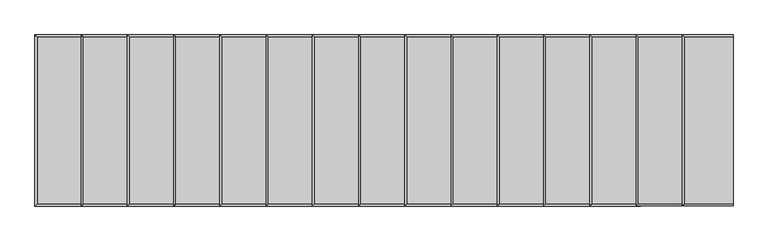
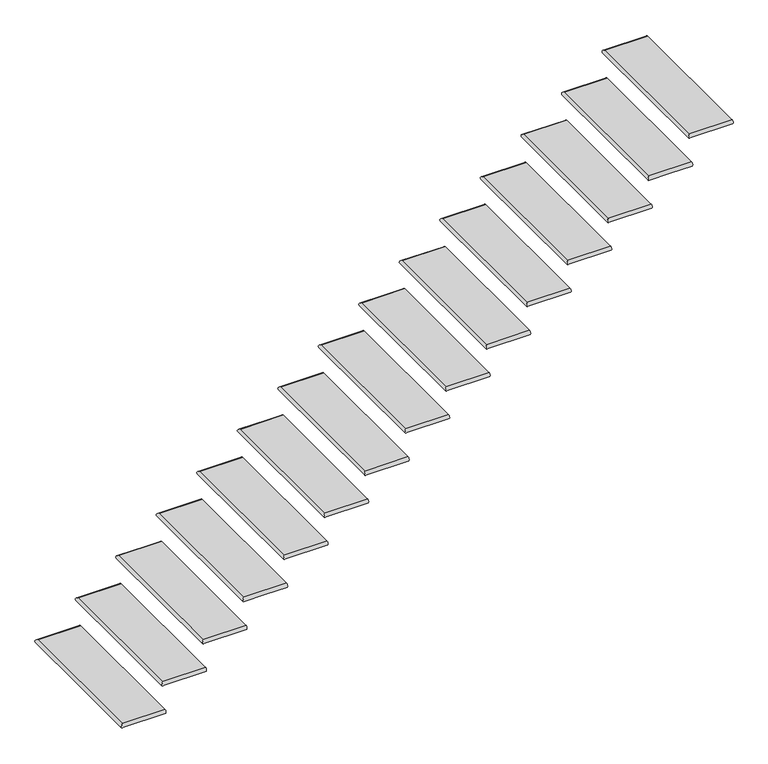
"""IFC4 building model written with IfcOpenShell, lengths in millimetres: stair flight geometry."""

from ifc_helpers import new_model, si_unit, frame, origin, place, context, project, spatial, circle_curve, ellipse_curve, source, transform, mapped, element, save
from ifc_brep_helpers import plane_surface, cylinder_surface, advanced_brep


def stair_flight_3500c2e6(model_context):
    return source(origin(), model_context, "Body", "AdvancedBrep", [
        advanced_brep(
        [(-27218.1481446, -8236.0871906, 165.1), (-27218.1481446, -8236.0871906, 190.5), (-27218.1481446, -7321.6871906, 190.5), (-27218.1481446, -7321.6871906, 165.1), (-26951.4481446, -8236.0871906, 190.5), (-26951.4481446, -7321.6871906, 190.5), (-26951.4481446, -7321.6871906, 165.1), (-26951.4481446, -8236.0871906, 165.1)],
        [
            (0, 1, ellipse_curve(frame((-27218.1481446, -8236.0871906, 177.8), z_axis=(-0.7071067811865464, 0.7071067811865488, 0.0), x_axis=(-0.7071067811865489, -0.707106781186546, 0.0)), 17.9605122, 12.7)),
            (1, 2),
            (2, 3, ellipse_curve(frame((-27218.1481446, -7321.6871906, 177.8), z_axis=(-0.7071067811865487, -0.7071067811865462, 0.0), x_axis=(0.7071067811865462, -0.707106781186549, 0.0)), 17.9605122, 12.7)),
            (3, 0),
            (4, 5),
            (5, 2),
            (1, 4),
            (6, 7),
            (7, 0),
            (3, 6),
            (4, 7, circle_curve(frame((-26951.4481446, -8236.0871906, 177.8), z_axis=(1.0, 0.0, 0.0), x_axis=(0.0, 1.0, 0.0)), 12.7)),
            (6, 5, circle_curve(frame((-26951.4481446, -7321.6871906, 177.8), z_axis=(1.0, 0.0, 0.0), x_axis=(0.0, -1.0, 0.0)), 12.7)),
        ],
        [
            cylinder_surface(frame((-27218.1481446, -8236.0871906, 177.8), z_axis=(0.0, -1.0, 0.0), x_axis=(1.0, 0.0, 0.0)), 12.7),
            plane_surface(frame((-27230.8481446, -7321.6871906, 190.5), z_axis=(0.0, 0.0, 1.0), x_axis=(-1.0, 0.0, 0.0))),
            plane_surface(frame((-27230.8481446, -7321.6871906, 165.1), z_axis=(0.0, 0.0, -1.0), x_axis=(1.0, 0.0, 0.0))),
            plane_surface(frame((-26951.4481446, -8236.0871906, 190.5), z_axis=(1.0, 0.0, 0.0), x_axis=(0.0, 0.0, -1.0))),
            cylinder_surface(frame((-26951.4481446, -8236.0871906, 177.8), z_axis=(1.0, 0.0, 0.0), x_axis=(0.0, 1.0, 0.0)), 12.7),
            cylinder_surface(frame((-27218.1481446, -7321.6871906, 177.8), z_axis=(-1.0, 0.0, 0.0), x_axis=(0.0, -1.0, 0.0)), 12.7),
        ],
        [
            (0, [[1, 2, 3, 4]]),
            (1, [[5, 6, -2, 7]]),
            (2, [[8, 9, -4, 10]]),
            (3, [[-5, 11, -8, 12]]),
            (4, [[-11, -7, -1, -9]]),
            (5, [[-3, -6, -12, -10]]),
        ],
    ),
        advanced_brep(
        [(-26697.4481446, -8236.0871906, 381.0), (-26697.4481446, -7321.6871906, 381.0), (-26964.1481446, -7321.6871906, 381.0), (-26964.1481446, -8236.0871906, 381.0), (-26697.4481446, -7321.6871906, 355.6), (-26697.4481446, -8236.0871906, 355.6), (-26964.1481446, -8236.0871906, 355.6), (-26964.1481446, -7321.6871906, 355.6)],
        [
            (0, 1),
            (1, 2),
            (2, 3),
            (3, 0),
            (4, 5),
            (5, 6),
            (6, 7),
            (7, 4),
            (0, 5, circle_curve(frame((-26697.4481446, -8236.0871906, 368.3), z_axis=(1.0, 0.0, 0.0), x_axis=(0.0, 1.0, 0.0)), 12.7)),
            (4, 1, circle_curve(frame((-26697.4481446, -7321.6871906, 368.3), z_axis=(1.0, 0.0, 0.0), x_axis=(0.0, -1.0, 0.0)), 12.7)),
            (3, 6, ellipse_curve(frame((-26964.1481446, -8236.0871906, 368.3), z_axis=(0.7071067811865464, -0.7071067811865488, 0.0), x_axis=(0.7071067811865487, 0.7071067811865464, 0.0)), 17.9605122, 12.7)),
            (2, 7, ellipse_curve(frame((-26964.1481446, -7321.6871906, 368.3), z_axis=(-0.7071067811865487, -0.7071067811865462, 0.0), x_axis=(0.7071067811865462, -0.707106781186549, 0.0)), 17.9605122, 12.7)),
        ],
        [
            plane_surface(frame((-26976.8481446, -7321.6871906, 381.0), z_axis=(0.0, 0.0, 1.0), x_axis=(-1.0, 0.0, 0.0))),
            plane_surface(frame((-26976.8481446, -7321.6871906, 355.6), z_axis=(0.0, 0.0, -1.0), x_axis=(1.0, 0.0, 0.0))),
            plane_surface(frame((-26697.4481446, -8236.0871906, 381.0), z_axis=(1.0, 0.0, 0.0), x_axis=(0.0, 0.0, -1.0))),
            cylinder_surface(frame((-26697.4481446, -8236.0871906, 368.3), z_axis=(1.0, 0.0, 0.0), x_axis=(0.0, 1.0, 0.0)), 12.7),
            cylinder_surface(frame((-26964.1481446, -8236.0871906, 368.3), z_axis=(0.0, -1.0, 0.0), x_axis=(1.0, 0.0, 0.0)), 12.7),
            cylinder_surface(frame((-26964.1481446, -7321.6871906, 368.3), z_axis=(-1.0, 0.0, 0.0), x_axis=(0.0, -1.0, 0.0)), 12.7),
        ],
        [
            (0, [[1, 2, 3, 4]]),
            (1, [[5, 6, 7, 8]]),
            (2, [[-1, 9, -5, 10]]),
            (3, [[-9, -4, 11, -6]]),
            (4, [[-11, -3, 12, -7]]),
            (5, [[-12, -2, -10, -8]]),
        ],
    ),
        advanced_brep(
        [(-26443.4481446, -8236.0871906, 571.5), (-26443.4481446, -7321.6871906, 571.5), (-26710.1481446, -7321.6871906, 571.5), (-26710.1481446, -8236.0871906, 571.5), (-26443.4481446, -7321.6871906, 546.1), (-26443.4481446, -8236.0871906, 546.1), (-26710.1481446, -8236.0871906, 546.1), (-26710.1481446, -7321.6871906, 546.1)],
        [
            (0, 1),
            (1, 2),
            (2, 3),
            (3, 0),
            (4, 5),
            (5, 6),
            (6, 7),
            (7, 4),
            (0, 5, circle_curve(frame((-26443.4481446, -8236.0871906, 558.8), z_axis=(1.0, 0.0, 0.0), x_axis=(0.0, 1.0, 0.0)), 12.7)),
            (4, 1, circle_curve(frame((-26443.4481446, -7321.6871906, 558.8), z_axis=(1.0, 0.0, 0.0), x_axis=(0.0, -1.0, 0.0)), 12.7)),
            (3, 6, ellipse_curve(frame((-26710.1481446, -8236.0871906, 558.8), z_axis=(0.7071067811865464, -0.7071067811865488, 0.0), x_axis=(0.7071067811865487, 0.7071067811865464, 0.0)), 17.9605122, 12.7)),
            (2, 7, ellipse_curve(frame((-26710.1481446, -7321.6871906, 558.8), z_axis=(-0.7071067811865487, -0.7071067811865462, 0.0), x_axis=(0.7071067811865462, -0.707106781186549, 0.0)), 17.9605122, 12.7)),
        ],
        [
            plane_surface(frame((-26722.8481446, -7321.6871906, 571.5), z_axis=(0.0, 0.0, 1.0), x_axis=(-1.0, 0.0, 0.0))),
            plane_surface(frame((-26722.8481446, -7321.6871906, 546.1), z_axis=(0.0, 0.0, -1.0), x_axis=(1.0, 0.0, 0.0))),
            plane_surface(frame((-26443.4481446, -8236.0871906, 571.5), z_axis=(1.0, 0.0, 0.0), x_axis=(0.0, 0.0, -1.0))),
            cylinder_surface(frame((-26443.4481446, -8236.0871906, 558.8), z_axis=(1.0, 0.0, 0.0), x_axis=(0.0, 1.0, 0.0)), 12.7),
            cylinder_surface(frame((-26710.1481446, -8236.0871906, 558.8), z_axis=(0.0, -1.0, 0.0), x_axis=(1.0, 0.0, 0.0)), 12.7),
            cylinder_surface(frame((-26710.1481446, -7321.6871906, 558.8), z_axis=(-1.0, 0.0, 0.0), x_axis=(0.0, -1.0, 0.0)), 12.7),
        ],
        [
            (0, [[1, 2, 3, 4]]),
            (1, [[5, 6, 7, 8]]),
            (2, [[-1, 9, -5, 10]]),
            (3, [[-9, -4, 11, -6]]),
            (4, [[-11, -3, 12, -7]]),
            (5, [[-12, -2, -10, -8]]),
        ],
    ),
        advanced_brep(
        [(-26189.4481446, -8236.0871906, 762.0), (-26189.4481446, -7321.6871906, 762.0), (-26456.1481446, -7321.6871906, 762.0), (-26456.1481446, -8236.0871906, 762.0), (-26189.4481446, -7321.6871906, 736.6), (-26189.4481446, -8236.0871906, 736.6), (-26456.1481446, -8236.0871906, 736.6), (-26456.1481446, -7321.6871906, 736.6)],
        [
            (0, 1),
            (1, 2),
            (2, 3),
            (3, 0),
            (4, 5),
            (5, 6),
            (6, 7),
            (7, 4),
            (0, 5, circle_curve(frame((-26189.4481446, -8236.0871906, 749.3), z_axis=(1.0, 0.0, 0.0), x_axis=(0.0, 1.0, 0.0)), 12.7)),
            (4, 1, circle_curve(frame((-26189.4481446, -7321.6871906, 749.3), z_axis=(1.0, 0.0, 0.0), x_axis=(0.0, -1.0, 0.0)), 12.7)),
            (3, 6, ellipse_curve(frame((-26456.1481446, -8236.0871906, 749.3), z_axis=(0.7071067811865464, -0.7071067811865488, 0.0), x_axis=(0.7071067811865487, 0.7071067811865464, 0.0)), 17.9605122, 12.7)),
            (2, 7, ellipse_curve(frame((-26456.1481446, -7321.6871906, 749.3), z_axis=(-0.7071067811865487, -0.7071067811865462, 0.0), x_axis=(0.7071067811865462, -0.707106781186549, 0.0)), 17.9605122, 12.7)),
        ],
        [
            plane_surface(frame((-26468.8481446, -7321.6871906, 762.0), z_axis=(0.0, 0.0, 1.0), x_axis=(-1.0, 0.0, 0.0))),
            plane_surface(frame((-26468.8481446, -7321.6871906, 736.6), z_axis=(0.0, 0.0, -1.0), x_axis=(1.0, 0.0, 0.0))),
            plane_surface(frame((-26189.4481446, -8236.0871906, 762.0), z_axis=(1.0, 0.0, 0.0), x_axis=(0.0, 0.0, -1.0))),
            cylinder_surface(frame((-26189.4481446, -8236.0871906, 749.3), z_axis=(1.0, 0.0, 0.0), x_axis=(0.0, 1.0, 0.0)), 12.7),
            cylinder_surface(frame((-26456.1481446, -8236.0871906, 749.3), z_axis=(0.0, -1.0, 0.0), x_axis=(1.0, 0.0, 0.0)), 12.7),
            cylinder_surface(frame((-26456.1481446, -7321.6871906, 749.3), z_axis=(-1.0, 0.0, 0.0), x_axis=(0.0, -1.0, 0.0)), 12.7),
        ],
        [
            (0, [[1, 2, 3, 4]]),
            (1, [[5, 6, 7, 8]]),
            (2, [[-1, 9, -5, 10]]),
            (3, [[-9, -4, 11, -6]]),
            (4, [[-11, -3, 12, -7]]),
            (5, [[-12, -2, -10, -8]]),
        ],
    ),
        advanced_brep(
        [(-25935.4481446, -8236.0871906, 952.5), (-25935.4481446, -7321.6871906, 952.5), (-26202.1481446, -7321.6871906, 952.5), (-26202.1481446, -8236.0871906, 952.5), (-25935.4481446, -7321.6871906, 927.1), (-25935.4481446, -8236.0871906, 927.1), (-26202.1481446, -8236.0871906, 927.1), (-26202.1481446, -7321.6871906, 927.1)],
        [
            (0, 1),
            (1, 2),
            (2, 3),
            (3, 0),
            (4, 5),
            (5, 6),
            (6, 7),
            (7, 4),
            (0, 5, circle_curve(frame((-25935.4481446, -8236.0871906, 939.8), z_axis=(1.0, 0.0, 0.0), x_axis=(0.0, 1.0, 0.0)), 12.7)),
            (4, 1, circle_curve(frame((-25935.4481446, -7321.6871906, 939.8), z_axis=(1.0, 0.0, 0.0), x_axis=(0.0, -1.0, 0.0)), 12.7)),
            (3, 6, ellipse_curve(frame((-26202.1481446, -8236.0871906, 939.8), z_axis=(0.7071067811865464, -0.7071067811865488, 0.0), x_axis=(0.7071067811865487, 0.7071067811865464, 0.0)), 17.9605122, 12.7)),
            (2, 7, ellipse_curve(frame((-26202.1481446, -7321.6871906, 939.8), z_axis=(-0.7071067811865487, -0.7071067811865462, 0.0), x_axis=(0.7071067811865462, -0.707106781186549, 0.0)), 17.9605122, 12.7)),
        ],
        [
            plane_surface(frame((-26214.8481446, -7321.6871906, 952.5), z_axis=(0.0, 0.0, 1.0), x_axis=(-1.0, 0.0, 0.0))),
            plane_surface(frame((-26214.8481446, -7321.6871906, 927.1), z_axis=(0.0, 0.0, -1.0), x_axis=(1.0, 0.0, 0.0))),
            plane_surface(frame((-25935.4481446, -8236.0871906, 952.5), z_axis=(1.0, 0.0, 0.0), x_axis=(0.0, 0.0, -1.0))),
            cylinder_surface(frame((-25935.4481446, -8236.0871906, 939.8), z_axis=(1.0, 0.0, 0.0), x_axis=(0.0, 1.0, 0.0)), 12.7),
            cylinder_surface(frame((-26202.1481446, -8236.0871906, 939.8), z_axis=(0.0, -1.0, 0.0), x_axis=(1.0, 0.0, 0.0)), 12.7),
            cylinder_surface(frame((-26202.1481446, -7321.6871906, 939.8), z_axis=(-1.0, 0.0, 0.0), x_axis=(0.0, -1.0, 0.0)), 12.7),
        ],
        [
            (0, [[1, 2, 3, 4]]),
            (1, [[5, 6, 7, 8]]),
            (2, [[-1, 9, -5, 10]]),
            (3, [[-9, -4, 11, -6]]),
            (4, [[-11, -3, 12, -7]]),
            (5, [[-12, -2, -10, -8]]),
        ],
    ),
        advanced_brep(
        [(-25681.4481446, -8236.0871906, 1143.0), (-25681.4481446, -7321.6871906, 1143.0), (-25948.1481446, -7321.6871906, 1143.0), (-25948.1481446, -8236.0871906, 1143.0), (-25681.4481446, -7321.6871906, 1117.6), (-25681.4481446, -8236.0871906, 1117.6), (-25948.1481446, -8236.0871906, 1117.6), (-25948.1481446, -7321.6871906, 1117.6)],
        [
            (0, 1),
            (1, 2),
            (2, 3),
            (3, 0),
            (4, 5),
            (5, 6),
            (6, 7),
            (7, 4),
            (0, 5, circle_curve(frame((-25681.4481446, -8236.0871906, 1130.3), z_axis=(1.0, 0.0, 0.0), x_axis=(0.0, 1.0, 0.0)), 12.7)),
            (4, 1, circle_curve(frame((-25681.4481446, -7321.6871906, 1130.3), z_axis=(1.0, 0.0, 0.0), x_axis=(0.0, -1.0, 0.0)), 12.7)),
            (3, 6, ellipse_curve(frame((-25948.1481446, -8236.0871906, 1130.3), z_axis=(0.7071067811865464, -0.7071067811865488, 0.0), x_axis=(0.7071067811865487, 0.7071067811865464, 0.0)), 17.9605122, 12.7)),
            (2, 7, ellipse_curve(frame((-25948.1481446, -7321.6871906, 1130.3), z_axis=(-0.7071067811865487, -0.7071067811865462, 0.0), x_axis=(0.7071067811865462, -0.707106781186549, 0.0)), 17.9605122, 12.7)),
        ],
        [
            plane_surface(frame((-25960.8481446, -7321.6871906, 1143.0), z_axis=(0.0, 0.0, 1.0), x_axis=(-1.0, 0.0, 0.0))),
            plane_surface(frame((-25960.8481446, -7321.6871906, 1117.6), z_axis=(0.0, 0.0, -1.0), x_axis=(1.0, 0.0, 0.0))),
            plane_surface(frame((-25681.4481446, -8236.0871906, 1143.0), z_axis=(1.0, 0.0, 0.0), x_axis=(0.0, 0.0, -1.0))),
            cylinder_surface(frame((-25681.4481446, -8236.0871906, 1130.3), z_axis=(1.0, 0.0, 0.0), x_axis=(0.0, 1.0, 0.0)), 12.7),
            cylinder_surface(frame((-25948.1481446, -8236.0871906, 1130.3), z_axis=(0.0, -1.0, 0.0), x_axis=(1.0, 0.0, 0.0)), 12.7),
            cylinder_surface(frame((-25948.1481446, -7321.6871906, 1130.3), z_axis=(-1.0, 0.0, 0.0), x_axis=(0.0, -1.0, 0.0)), 12.7),
        ],
        [
            (0, [[1, 2, 3, 4]]),
            (1, [[5, 6, 7, 8]]),
            (2, [[-1, 9, -5, 10]]),
            (3, [[-9, -4, 11, -6]]),
            (4, [[-11, -3, 12, -7]]),
            (5, [[-12, -2, -10, -8]]),
        ],
    ),
        advanced_brep(
        [(-25427.4481446, -8236.0871906, 1333.5), (-25427.4481446, -7321.6871906, 1333.5), (-25694.1481446, -7321.6871906, 1333.5), (-25694.1481446, -8236.0871906, 1333.5), (-25427.4481446, -7321.6871906, 1308.1), (-25427.4481446, -8236.0871906, 1308.1), (-25694.1481446, -8236.0871906, 1308.1), (-25694.1481446, -7321.6871906, 1308.1)],
        [
            (0, 1),
            (1, 2),
            (2, 3),
            (3, 0),
            (4, 5),
            (5, 6),
            (6, 7),
            (7, 4),
            (0, 5, circle_curve(frame((-25427.4481446, -8236.0871906, 1320.8), z_axis=(1.0, 0.0, 0.0), x_axis=(0.0, 1.0, 0.0)), 12.7)),
            (4, 1, circle_curve(frame((-25427.4481446, -7321.6871906, 1320.8), z_axis=(1.0, 0.0, 0.0), x_axis=(0.0, -1.0, 0.0)), 12.7)),
            (3, 6, ellipse_curve(frame((-25694.1481446, -8236.0871906, 1320.8), z_axis=(0.7071067811865464, -0.7071067811865488, 0.0), x_axis=(0.7071067811865487, 0.7071067811865464, 0.0)), 17.9605122, 12.7)),
            (2, 7, ellipse_curve(frame((-25694.1481446, -7321.6871906, 1320.8), z_axis=(-0.7071067811865487, -0.7071067811865462, 0.0), x_axis=(0.7071067811865462, -0.707106781186549, 0.0)), 17.9605122, 12.7)),
        ],
        [
            plane_surface(frame((-25706.8481446, -7321.6871906, 1333.5), z_axis=(0.0, 0.0, 1.0), x_axis=(-1.0, 0.0, 0.0))),
            plane_surface(frame((-25706.8481446, -7321.6871906, 1308.1), z_axis=(0.0, 0.0, -1.0), x_axis=(1.0, 0.0, 0.0))),
            plane_surface(frame((-25427.4481446, -8236.0871906, 1333.5), z_axis=(1.0, 0.0, 0.0), x_axis=(0.0, 0.0, -1.0))),
            cylinder_surface(frame((-25427.4481446, -8236.0871906, 1320.8), z_axis=(1.0, 0.0, 0.0), x_axis=(0.0, 1.0, 0.0)), 12.7),
            cylinder_surface(frame((-25694.1481446, -8236.0871906, 1320.8), z_axis=(0.0, -1.0, 0.0), x_axis=(1.0, 0.0, 0.0)), 12.7),
            cylinder_surface(frame((-25694.1481446, -7321.6871906, 1320.8), z_axis=(-1.0, 0.0, 0.0), x_axis=(0.0, -1.0, 0.0)), 12.7),
        ],
        [
            (0, [[1, 2, 3, 4]]),
            (1, [[5, 6, 7, 8]]),
            (2, [[-1, 9, -5, 10]]),
            (3, [[-9, -4, 11, -6]]),
            (4, [[-11, -3, 12, -7]]),
            (5, [[-12, -2, -10, -8]]),
        ],
    ),
        advanced_brep(
        [(-25173.4481446, -8236.0871906, 1524.0), (-25173.4481446, -7321.6871906, 1524.0), (-25440.1481446, -7321.6871906, 1524.0), (-25440.1481446, -8236.0871906, 1524.0), (-25173.4481446, -7321.6871906, 1498.6), (-25173.4481446, -8236.0871906, 1498.6), (-25440.1481446, -8236.0871906, 1498.6), (-25440.1481446, -7321.6871906, 1498.6)],
        [
            (0, 1),
            (1, 2),
            (2, 3),
            (3, 0),
            (4, 5),
            (5, 6),
            (6, 7),
            (7, 4),
            (0, 5, circle_curve(frame((-25173.4481446, -8236.0871906, 1511.3), z_axis=(1.0, 0.0, 0.0), x_axis=(0.0, 1.0, 0.0)), 12.7)),
            (4, 1, circle_curve(frame((-25173.4481446, -7321.6871906, 1511.3), z_axis=(1.0, 0.0, 0.0), x_axis=(0.0, -1.0, 0.0)), 12.7)),
            (3, 6, ellipse_curve(frame((-25440.1481446, -8236.0871906, 1511.3), z_axis=(0.7071067811865464, -0.7071067811865488, 0.0), x_axis=(0.7071067811865487, 0.7071067811865464, 0.0)), 17.9605122, 12.7)),
            (2, 7, ellipse_curve(frame((-25440.1481446, -7321.6871906, 1511.3), z_axis=(-0.7071067811865487, -0.7071067811865462, 0.0), x_axis=(0.7071067811865462, -0.707106781186549, 0.0)), 17.9605122, 12.7)),
        ],
        [
            plane_surface(frame((-25452.8481446, -7321.6871906, 1524.0), z_axis=(0.0, 0.0, 1.0), x_axis=(-1.0, 0.0, 0.0))),
            plane_surface(frame((-25452.8481446, -7321.6871906, 1498.6), z_axis=(0.0, 0.0, -1.0), x_axis=(1.0, 0.0, 0.0))),
            plane_surface(frame((-25173.4481446, -8236.0871906, 1524.0), z_axis=(1.0, 0.0, 0.0), x_axis=(0.0, 0.0, -1.0))),
            cylinder_surface(frame((-25173.4481446, -8236.0871906, 1511.3), z_axis=(1.0, 0.0, 0.0), x_axis=(0.0, 1.0, 0.0)), 12.7),
            cylinder_surface(frame((-25440.1481446, -8236.0871906, 1511.3), z_axis=(0.0, -1.0, 0.0), x_axis=(1.0, 0.0, 0.0)), 12.7),
            cylinder_surface(frame((-25440.1481446, -7321.6871906, 1511.3), z_axis=(-1.0, 0.0, 0.0), x_axis=(0.0, -1.0, 0.0)), 12.7),
        ],
        [
            (0, [[1, 2, 3, 4]]),
            (1, [[5, 6, 7, 8]]),
            (2, [[-1, 9, -5, 10]]),
            (3, [[-9, -4, 11, -6]]),
            (4, [[-11, -3, 12, -7]]),
            (5, [[-12, -2, -10, -8]]),
        ],
    ),
        advanced_brep(
        [(-24919.4481446, -8236.0871906, 1714.5), (-24919.4481446, -7321.6871906, 1714.5), (-25186.1481446, -7321.6871906, 1714.5), (-25186.1481446, -8236.0871906, 1714.5), (-24919.4481446, -7321.6871906, 1689.1), (-24919.4481446, -8236.0871906, 1689.1), (-25186.1481446, -8236.0871906, 1689.1), (-25186.1481446, -7321.6871906, 1689.1)],
        [
            (0, 1),
            (1, 2),
            (2, 3),
            (3, 0),
            (4, 5),
            (5, 6),
            (6, 7),
            (7, 4),
            (0, 5, circle_curve(frame((-24919.4481446, -8236.0871906, 1701.8), z_axis=(1.0, 0.0, 0.0), x_axis=(0.0, 1.0, 0.0)), 12.7)),
            (4, 1, circle_curve(frame((-24919.4481446, -7321.6871906, 1701.8), z_axis=(1.0, 0.0, 0.0), x_axis=(0.0, -1.0, 0.0)), 12.7)),
            (3, 6, ellipse_curve(frame((-25186.1481446, -8236.0871906, 1701.8), z_axis=(0.7071067811865464, -0.7071067811865488, 0.0), x_axis=(0.7071067811865487, 0.7071067811865464, 0.0)), 17.9605122, 12.7)),
            (2, 7, ellipse_curve(frame((-25186.1481446, -7321.6871906, 1701.8), z_axis=(-0.7071067811865487, -0.7071067811865462, 0.0), x_axis=(0.7071067811865462, -0.707106781186549, 0.0)), 17.9605122, 12.7)),
        ],
        [
            plane_surface(frame((-25198.8481446, -7321.6871906, 1714.5), z_axis=(0.0, 0.0, 1.0), x_axis=(-1.0, 0.0, 0.0))),
            plane_surface(frame((-25198.8481446, -7321.6871906, 1689.1), z_axis=(0.0, 0.0, -1.0), x_axis=(1.0, 0.0, 0.0))),
            plane_surface(frame((-24919.4481446, -8236.0871906, 1714.5), z_axis=(1.0, 0.0, 0.0), x_axis=(0.0, 0.0, -1.0))),
            cylinder_surface(frame((-24919.4481446, -8236.0871906, 1701.8), z_axis=(1.0, 0.0, 0.0), x_axis=(0.0, 1.0, 0.0)), 12.7),
            cylinder_surface(frame((-25186.1481446, -8236.0871906, 1701.8), z_axis=(0.0, -1.0, 0.0), x_axis=(1.0, 0.0, 0.0)), 12.7),
            cylinder_surface(frame((-25186.1481446, -7321.6871906, 1701.8), z_axis=(-1.0, 0.0, 0.0), x_axis=(0.0, -1.0, 0.0)), 12.7),
        ],
        [
            (0, [[1, 2, 3, 4]]),
            (1, [[5, 6, 7, 8]]),
            (2, [[-1, 9, -5, 10]]),
            (3, [[-9, -4, 11, -6]]),
            (4, [[-11, -3, 12, -7]]),
            (5, [[-12, -2, -10, -8]]),
        ],
    ),
        advanced_brep(
        [(-24665.4481446, -8236.0871906, 1905.0), (-24665.4481446, -7321.6871906, 1905.0), (-24932.1481446, -7321.6871906, 1905.0), (-24932.1481446, -8236.0871906, 1905.0), (-24665.4481446, -7321.6871906, 1879.6), (-24665.4481446, -8236.0871906, 1879.6), (-24932.1481446, -8236.0871906, 1879.6), (-24932.1481446, -7321.6871906, 1879.6)],
        [
            (0, 1),
            (1, 2),
            (2, 3),
            (3, 0),
            (4, 5),
            (5, 6),
            (6, 7),
            (7, 4),
            (0, 5, circle_curve(frame((-24665.4481446, -8236.0871906, 1892.3), z_axis=(1.0, 0.0, 0.0), x_axis=(0.0, 1.0, 0.0)), 12.7)),
            (4, 1, circle_curve(frame((-24665.4481446, -7321.6871906, 1892.3), z_axis=(1.0, 0.0, 0.0), x_axis=(0.0, -1.0, 0.0)), 12.7)),
            (3, 6, ellipse_curve(frame((-24932.1481446, -8236.0871906, 1892.3), z_axis=(0.7071067811865464, -0.7071067811865488, 0.0), x_axis=(0.7071067811865487, 0.7071067811865464, 0.0)), 17.9605122, 12.7)),
            (2, 7, ellipse_curve(frame((-24932.1481446, -7321.6871906, 1892.3), z_axis=(-0.7071067811865487, -0.7071067811865462, 0.0), x_axis=(0.7071067811865462, -0.707106781186549, 0.0)), 17.9605122, 12.7)),
        ],
        [
            plane_surface(frame((-24944.8481446, -7321.6871906, 1905.0), z_axis=(0.0, 0.0, 1.0), x_axis=(-1.0, 0.0, 0.0))),
            plane_surface(frame((-24944.8481446, -7321.6871906, 1879.6), z_axis=(0.0, 0.0, -1.0), x_axis=(1.0, 0.0, 0.0))),
            plane_surface(frame((-24665.4481446, -8236.0871906, 1905.0), z_axis=(1.0, 0.0, 0.0), x_axis=(0.0, 0.0, -1.0))),
            cylinder_surface(frame((-24665.4481446, -8236.0871906, 1892.3), z_axis=(1.0, 0.0, 0.0), x_axis=(0.0, 1.0, 0.0)), 12.7),
            cylinder_surface(frame((-24932.1481446, -8236.0871906, 1892.3), z_axis=(0.0, -1.0, 0.0), x_axis=(1.0, 0.0, 0.0)), 12.7),
            cylinder_surface(frame((-24932.1481446, -7321.6871906, 1892.3), z_axis=(-1.0, 0.0, 0.0), x_axis=(0.0, -1.0, 0.0)), 12.7),
        ],
        [
            (0, [[1, 2, 3, 4]]),
            (1, [[5, 6, 7, 8]]),
            (2, [[-1, 9, -5, 10]]),
            (3, [[-9, -4, 11, -6]]),
            (4, [[-11, -3, 12, -7]]),
            (5, [[-12, -2, -10, -8]]),
        ],
    ),
        advanced_brep(
        [(-24411.4481446, -8236.0871906, 2095.5), (-24411.4481446, -7321.6871906, 2095.5), (-24678.1481446, -7321.6871906, 2095.5), (-24678.1481446, -8236.0871906, 2095.5), (-24411.4481446, -7321.6871906, 2070.1), (-24411.4481446, -8236.0871906, 2070.1), (-24678.1481446, -8236.0871906, 2070.1), (-24678.1481446, -7321.6871906, 2070.1)],
        [
            (0, 1),
            (1, 2),
            (2, 3),
            (3, 0),
            (4, 5),
            (5, 6),
            (6, 7),
            (7, 4),
            (0, 5, circle_curve(frame((-24411.4481446, -8236.0871906, 2082.8), z_axis=(1.0, 0.0, 0.0), x_axis=(0.0, 1.0, 0.0)), 12.7)),
            (4, 1, circle_curve(frame((-24411.4481446, -7321.6871906, 2082.8), z_axis=(1.0, 0.0, 0.0), x_axis=(0.0, -1.0, 0.0)), 12.7)),
            (3, 6, ellipse_curve(frame((-24678.1481446, -8236.0871906, 2082.8), z_axis=(0.7071067811865464, -0.7071067811865488, 0.0), x_axis=(0.7071067811865487, 0.7071067811865464, 0.0)), 17.9605122, 12.7)),
            (2, 7, ellipse_curve(frame((-24678.1481446, -7321.6871906, 2082.8), z_axis=(-0.7071067811865487, -0.7071067811865462, 0.0), x_axis=(0.7071067811865462, -0.707106781186549, 0.0)), 17.9605122, 12.7)),
        ],
        [
            plane_surface(frame((-24690.8481446, -7321.6871906, 2095.5), z_axis=(0.0, 0.0, 1.0), x_axis=(-1.0, 0.0, 0.0))),
            plane_surface(frame((-24690.8481446, -7321.6871906, 2070.1), z_axis=(0.0, 0.0, -1.0), x_axis=(1.0, 0.0, 0.0))),
            plane_surface(frame((-24411.4481446, -8236.0871906, 2095.5), z_axis=(1.0, 0.0, 0.0), x_axis=(0.0, 0.0, -1.0))),
            cylinder_surface(frame((-24411.4481446, -8236.0871906, 2082.8), z_axis=(1.0, 0.0, 0.0), x_axis=(0.0, 1.0, 0.0)), 12.7),
            cylinder_surface(frame((-24678.1481446, -8236.0871906, 2082.8), z_axis=(0.0, -1.0, 0.0), x_axis=(1.0, 0.0, 0.0)), 12.7),
            cylinder_surface(frame((-24678.1481446, -7321.6871906, 2082.8), z_axis=(-1.0, 0.0, 0.0), x_axis=(0.0, -1.0, 0.0)), 12.7),
        ],
        [
            (0, [[1, 2, 3, 4]]),
            (1, [[5, 6, 7, 8]]),
            (2, [[-1, 9, -5, 10]]),
            (3, [[-9, -4, 11, -6]]),
            (4, [[-11, -3, 12, -7]]),
            (5, [[-12, -2, -10, -8]]),
        ],
    ),
        advanced_brep(
        [(-24157.4481446, -8236.0871906, 2286.0), (-24157.4481446, -7321.6871906, 2286.0), (-24424.1481446, -7321.6871906, 2286.0), (-24424.1481446, -8236.0871906, 2286.0), (-24157.4481446, -7321.6871906, 2260.6), (-24157.4481446, -8236.0871906, 2260.6), (-24424.1481446, -8236.0871906, 2260.6), (-24424.1481446, -7321.6871906, 2260.6)],
        [
            (0, 1),
            (1, 2),
            (2, 3),
            (3, 0),
            (4, 5),
            (5, 6),
            (6, 7),
            (7, 4),
            (0, 5, circle_curve(frame((-24157.4481446, -8236.0871906, 2273.3), z_axis=(1.0, 0.0, 0.0), x_axis=(0.0, 1.0, 0.0)), 12.7)),
            (4, 1, circle_curve(frame((-24157.4481446, -7321.6871906, 2273.3), z_axis=(1.0, 0.0, 0.0), x_axis=(0.0, -1.0, 0.0)), 12.7)),
            (3, 6, ellipse_curve(frame((-24424.1481446, -8236.0871906, 2273.3), z_axis=(0.7071067811865464, -0.7071067811865488, 0.0), x_axis=(0.7071067811865487, 0.7071067811865464, 0.0)), 17.9605122, 12.7)),
            (2, 7, ellipse_curve(frame((-24424.1481446, -7321.6871906, 2273.3), z_axis=(-0.7071067811865487, -0.7071067811865462, 0.0), x_axis=(0.7071067811865462, -0.707106781186549, 0.0)), 17.9605122, 12.7)),
        ],
        [
            plane_surface(frame((-24436.8481446, -7321.6871906, 2286.0), z_axis=(0.0, 0.0, 1.0), x_axis=(-1.0, 0.0, 0.0))),
            plane_surface(frame((-24436.8481446, -7321.6871906, 2260.6), z_axis=(0.0, 0.0, -1.0), x_axis=(1.0, 0.0, 0.0))),
            plane_surface(frame((-24157.4481446, -8236.0871906, 2286.0), z_axis=(1.0, 0.0, 0.0), x_axis=(0.0, 0.0, -1.0))),
            cylinder_surface(frame((-24157.4481446, -8236.0871906, 2273.3), z_axis=(1.0, 0.0, 0.0), x_axis=(0.0, 1.0, 0.0)), 12.7),
            cylinder_surface(frame((-24424.1481446, -8236.0871906, 2273.3), z_axis=(0.0, -1.0, 0.0), x_axis=(1.0, 0.0, 0.0)), 12.7),
            cylinder_surface(frame((-24424.1481446, -7321.6871906, 2273.3), z_axis=(-1.0, 0.0, 0.0), x_axis=(0.0, -1.0, 0.0)), 12.7),
        ],
        [
            (0, [[1, 2, 3, 4]]),
            (1, [[5, 6, 7, 8]]),
            (2, [[-1, 9, -5, 10]]),
            (3, [[-9, -4, 11, -6]]),
            (4, [[-11, -3, 12, -7]]),
            (5, [[-12, -2, -10, -8]]),
        ],
    ),
        advanced_brep(
        [(-23903.4481446, -8236.0871906, 2476.5), (-23903.4481446, -7321.6871906, 2476.5), (-24170.1481446, -7321.6871906, 2476.5), (-24170.1481446, -8236.0871906, 2476.5), (-23903.4481446, -7321.6871906, 2451.1), (-23903.4481446, -8236.0871906, 2451.1), (-24170.1481446, -8236.0871906, 2451.1), (-24170.1481446, -7321.6871906, 2451.1)],
        [
            (0, 1),
            (1, 2),
            (2, 3),
            (3, 0),
            (4, 5),
            (5, 6),
            (6, 7),
            (7, 4),
            (0, 5, circle_curve(frame((-23903.4481446, -8236.0871906, 2463.8), z_axis=(1.0, 0.0, 0.0), x_axis=(0.0, 1.0, 0.0)), 12.7)),
            (4, 1, circle_curve(frame((-23903.4481446, -7321.6871906, 2463.8), z_axis=(1.0, 0.0, 0.0), x_axis=(0.0, -1.0, 0.0)), 12.7)),
            (3, 6, ellipse_curve(frame((-24170.1481446, -8236.0871906, 2463.8), z_axis=(0.7071067811865464, -0.7071067811865488, 0.0), x_axis=(0.7071067811865487, 0.7071067811865464, 0.0)), 17.9605122, 12.7)),
            (2, 7, ellipse_curve(frame((-24170.1481446, -7321.6871906, 2463.8), z_axis=(-0.7071067811865487, -0.7071067811865462, 0.0), x_axis=(0.7071067811865462, -0.707106781186549, 0.0)), 17.9605122, 12.7)),
        ],
        [
            plane_surface(frame((-24182.8481446, -7321.6871906, 2476.5), z_axis=(0.0, 0.0, 1.0), x_axis=(-1.0, 0.0, 0.0))),
            plane_surface(frame((-24182.8481446, -7321.6871906, 2451.1), z_axis=(0.0, 0.0, -1.0), x_axis=(1.0, 0.0, 0.0))),
            plane_surface(frame((-23903.4481446, -8236.0871906, 2476.5), z_axis=(1.0, 0.0, 0.0), x_axis=(0.0, 0.0, -1.0))),
            cylinder_surface(frame((-23903.4481446, -8236.0871906, 2463.8), z_axis=(1.0, 0.0, 0.0), x_axis=(0.0, 1.0, 0.0)), 12.7),
            cylinder_surface(frame((-24170.1481446, -8236.0871906, 2463.8), z_axis=(0.0, -1.0, 0.0), x_axis=(1.0, 0.0, 0.0)), 12.7),
            cylinder_surface(frame((-24170.1481446, -7321.6871906, 2463.8), z_axis=(-1.0, 0.0, 0.0), x_axis=(0.0, -1.0, 0.0)), 12.7),
        ],
        [
            (0, [[1, 2, 3, 4]]),
            (1, [[5, 6, 7, 8]]),
            (2, [[-1, 9, -5, 10]]),
            (3, [[-9, -4, 11, -6]]),
            (4, [[-11, -3, 12, -7]]),
            (5, [[-12, -2, -10, -8]]),
        ],
    ),
        advanced_brep(
        [(-23649.4481446, -8236.0871906, 2667.0), (-23649.4481446, -7321.6871906, 2667.0), (-23916.1481446, -7321.6871906, 2667.0), (-23916.1481446, -8236.0871906, 2667.0), (-23649.4481446, -7321.6871906, 2641.6), (-23649.4481446, -8236.0871906, 2641.6), (-23916.1481446, -8236.0871906, 2641.6), (-23916.1481446, -7321.6871906, 2641.6)],
        [
            (0, 1),
            (1, 2),
            (2, 3),
            (3, 0),
            (4, 5),
            (5, 6),
            (6, 7),
            (7, 4),
            (0, 5, circle_curve(frame((-23649.4481446, -8236.0871906, 2654.3), z_axis=(1.0, 0.0, 0.0), x_axis=(0.0, 1.0, 0.0)), 12.7)),
            (4, 1, circle_curve(frame((-23649.4481446, -7321.6871906, 2654.3), z_axis=(1.0, 0.0, 0.0), x_axis=(0.0, -1.0, 0.0)), 12.7)),
            (3, 6, ellipse_curve(frame((-23916.1481446, -8236.0871906, 2654.3), z_axis=(0.7071067811865464, -0.7071067811865488, 0.0), x_axis=(0.7071067811865487, 0.7071067811865464, 0.0)), 17.9605122, 12.7)),
            (2, 7, ellipse_curve(frame((-23916.1481446, -7321.6871906, 2654.3), z_axis=(-0.7071067811865487, -0.7071067811865462, 0.0), x_axis=(0.7071067811865462, -0.707106781186549, 0.0)), 17.9605122, 12.7)),
        ],
        [
            plane_surface(frame((-23928.8481446, -7321.6871906, 2667.0), z_axis=(0.0, 0.0, 1.0), x_axis=(-1.0, 0.0, 0.0))),
            plane_surface(frame((-23928.8481446, -7321.6871906, 2641.6), z_axis=(0.0, 0.0, -1.0), x_axis=(1.0, 0.0, 0.0))),
            plane_surface(frame((-23649.4481446, -8236.0871906, 2667.0), z_axis=(1.0, 0.0, 0.0), x_axis=(0.0, 0.0, -1.0))),
            cylinder_surface(frame((-23649.4481446, -8236.0871906, 2654.3), z_axis=(1.0, 0.0, 0.0), x_axis=(0.0, 1.0, 0.0)), 12.7),
            cylinder_surface(frame((-23916.1481446, -8236.0871906, 2654.3), z_axis=(0.0, -1.0, 0.0), x_axis=(1.0, 0.0, 0.0)), 12.7),
            cylinder_surface(frame((-23916.1481446, -7321.6871906, 2654.3), z_axis=(-1.0, 0.0, 0.0), x_axis=(0.0, -1.0, 0.0)), 12.7),
        ],
        [
            (0, [[1, 2, 3, 4]]),
            (1, [[5, 6, 7, 8]]),
            (2, [[-1, 9, -5, 10]]),
            (3, [[-9, -4, 11, -6]]),
            (4, [[-11, -3, 12, -7]]),
            (5, [[-12, -2, -10, -8]]),
        ],
    ),
        advanced_brep(
        [(-23395.4481446, -8236.0871906, 2857.5), (-23395.4481446, -7321.6871906, 2857.5), (-23662.1481446, -7321.6871906, 2857.5), (-23662.1481446, -8236.0871906, 2857.5), (-23395.4481446, -7321.6871906, 2832.1), (-23395.4481446, -8236.0871906, 2832.1), (-23662.1481446, -8236.0871906, 2832.1), (-23662.1481446, -7321.6871906, 2832.1)],
        [
            (0, 1),
            (1, 2),
            (2, 3),
            (3, 0),
            (4, 5),
            (5, 6),
            (6, 7),
            (7, 4),
            (0, 5, circle_curve(frame((-23395.4481446, -8236.0871906, 2844.8), z_axis=(1.0, 0.0, 0.0), x_axis=(0.0, 1.0, 0.0)), 12.7)),
            (4, 1, circle_curve(frame((-23395.4481446, -7321.6871906, 2844.8), z_axis=(1.0, 0.0, 0.0), x_axis=(0.0, -1.0, 0.0)), 12.7)),
            (3, 6, ellipse_curve(frame((-23662.1481446, -8236.0871906, 2844.8), z_axis=(0.7071067811865464, -0.7071067811865488, 0.0), x_axis=(0.7071067811865487, 0.7071067811865464, 0.0)), 17.9605122, 12.7)),
            (2, 7, ellipse_curve(frame((-23662.1481446, -7321.6871906, 2844.8), z_axis=(-0.7071067811865487, -0.7071067811865462, 0.0), x_axis=(0.7071067811865462, -0.707106781186549, 0.0)), 17.9605122, 12.7)),
        ],
        [
            plane_surface(frame((-23674.8481446, -7321.6871906, 2857.5), z_axis=(0.0, 0.0, 1.0), x_axis=(-1.0, 0.0, 0.0))),
            plane_surface(frame((-23674.8481446, -7321.6871906, 2832.1), z_axis=(0.0, 0.0, -1.0), x_axis=(1.0, 0.0, 0.0))),
            plane_surface(frame((-23395.4481446, -8236.0871906, 2857.5), z_axis=(1.0, 0.0, 0.0), x_axis=(0.0, 0.0, -1.0))),
            cylinder_surface(frame((-23395.4481446, -8236.0871906, 2844.8), z_axis=(1.0, 0.0, 0.0), x_axis=(0.0, 1.0, 0.0)), 12.7),
            cylinder_surface(frame((-23662.1481446, -8236.0871906, 2844.8), z_axis=(0.0, -1.0, 0.0), x_axis=(1.0, 0.0, 0.0)), 12.7),
            cylinder_surface(frame((-23662.1481446, -7321.6871906, 2844.8), z_axis=(-1.0, 0.0, 0.0), x_axis=(0.0, -1.0, 0.0)), 12.7),
        ],
        [
            (0, [[1, 2, 3, 4]]),
            (1, [[5, 6, 7, 8]]),
            (2, [[-1, 9, -5, 10]]),
            (3, [[-9, -4, 11, -6]]),
            (4, [[-11, -3, 12, -7]]),
            (5, [[-12, -2, -10, -8]]),
        ],
    ),
    ])


if __name__ == "__main__":
    model = new_model("IFC4")
    model_context = context("Model", 3, world=origin())
    ifc_project = project(units=[si_unit("LENGTHUNIT", "METRE", prefix="MILLI")], contexts=[model_context])
    site = spatial("IfcSite", under=ifc_project)
    building = spatial("IfcBuilding", under=site)
    placement = place(None, origin())
    stair_flight_shape = stair_flight_3500c2e6(model_context)
    element("IfcStairFlight", 1, at=placement, inside=building, context=model_context, shape_type="MappedRepresentation", body=[
        mapped(stair_flight_shape, transform((0.0, 0.0, 0.0), x_axis=(1.0, 0.0, 0.0), y_axis=(0.0, 1.0, 0.0), z_axis=(0.0, 0.0, 1.0))),
    ])
    save(model, "model.ifc")

# Revit data of these elements
# Element 1 (IfcStairFlight)
#   Materials on its faces: "Wood - Cherry"
# Materials
#   "Wood - Cherry": class "Unassigned", colour RGB 226 177 128, transparency 0
